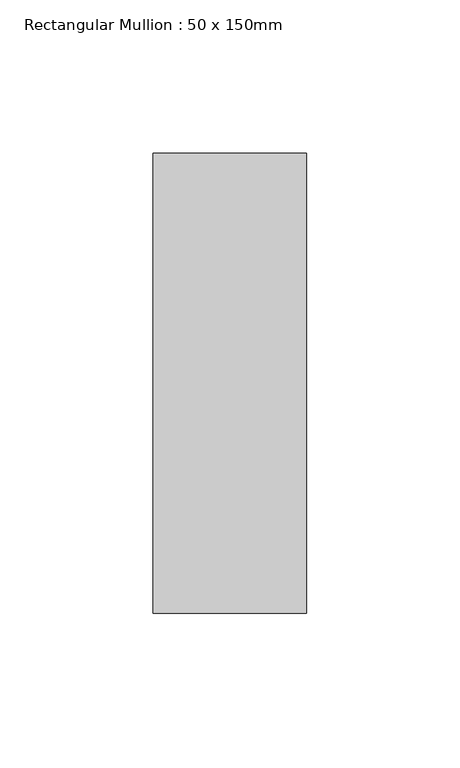
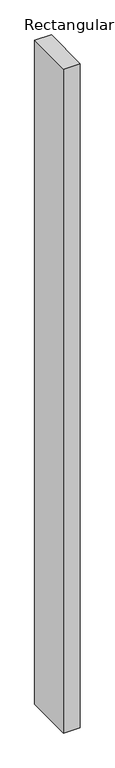
"""IFC4 building model written with IfcOpenShell, lengths in millimetres: member geometry, Rectangular Mullion : 50 x 150mm."""

import ifcopenshell
import ifcopenshell.guid

model = None  # the IFC model being written
_history = None  # IfcOwnerHistory: only IFC2X3 demands one
_inside = {}  # id of a spatial element -> (the spatial element, [elements in it])
_under = {}  # id of a project, library or spatial element -> (it, [spatial elements below it])
_declared = {}  # id of a project -> (the project, [libraries it declares])
_typed = {}  # id of a type object -> (the type object, [elements of that type])
_made_of = {}  # id of a material, layer set ... -> (it, [elements and type objects made of it])


def new_model(schema):
    """Start an empty IFC model of exactly this schema.

    Asked for "IFC4X3", IfcOpenShell would pick the latest addendum, in which some entities
    have other attributes; the version numbers below select the first issue.
    IFC2X3 requires an IfcOwnerHistory on every rooted entity: one is made here for all.
    """
    global model, _history
    if schema == "IFC4X3":
        model = ifcopenshell.file(schema_version=(4, 3, 0, 0))
    else:
        model = ifcopenshell.file(schema=schema)
    _inside.clear()
    _under.clear()
    _declared.clear()
    _typed.clear()
    _made_of.clear()
    _history = None
    if model.schema == "IFC2X3":
        org = make("IfcOrganization", Name="unknown")
        user = make(
            "IfcPersonAndOrganization",
            ThePerson=make("IfcPerson", FamilyName="unknown"),
            TheOrganization=org,
        )
        app = make(
            "IfcApplication",
            ApplicationDeveloper=org,
            Version="unknown",
            ApplicationFullName="unknown",
            ApplicationIdentifier="unknown",
        )
        _history = make(
            "IfcOwnerHistory",
            OwningUser=user,
            OwningApplication=app,
            ChangeAction="ADDED",
            CreationDate=0,
        )
    return model


def make(cls, **values):
    """One entity of the class cls with the attributes given. An attribute that is None is left unset."""
    return model.create_entity(
        cls, **{name: value for name, value in values.items() if value is not None}
    )


def rooted(cls, **values):
    """An entity with a GlobalId (a new one), such as an element, a storey or a relation."""
    return make(cls, GlobalId=ifcopenshell.guid.new(), OwnerHistory=_history, **values)


def si_unit(unit_type, name, prefix=None):
    """IfcSIUnit, for example si_unit("LENGTHUNIT", "METRE", prefix="MILLI")."""
    return make("IfcSIUnit", UnitType=unit_type, Prefix=prefix, Name=name)


def assignment(units):
    """IfcUnitAssignment: the units of a project."""
    return None if units is None else make("IfcUnitAssignment", Units=units)


def point(xyz):
    """IfcCartesianPoint."""
    return None if xyz is None else make("IfcCartesianPoint", Coordinates=xyz)


def direction(xyz):
    """IfcDirection."""
    return None if xyz is None else make("IfcDirection", DirectionRatios=xyz)


def frame(location, z_axis=None, x_axis=None):
    """IfcAxis2Placement3D, a coordinate frame: its origin and axes. An axis left out is left unset."""
    return make(
        "IfcAxis2Placement3D",
        Location=point(location),
        Axis=direction(z_axis),
        RefDirection=direction(x_axis),
    )


def origin():
    """The frame at (0, 0, 0) with its axes left unset."""
    return frame((0.0, 0.0, 0.0))


def place(relative_to, where):
    """IfcLocalPlacement: puts the frame where relative to a parent placement (None: the world)."""
    return make(
        "IfcLocalPlacement", PlacementRelTo=relative_to, RelativePlacement=where
    )


def context(
    kind, dimensions, precision=None, world=None, true_north=None, identifier=None
):
    """IfcGeometricRepresentationContext, for example the 3D "Model" context."""
    return make(
        "IfcGeometricRepresentationContext",
        ContextIdentifier=identifier,
        ContextType=kind,
        CoordinateSpaceDimension=dimensions,
        Precision=precision,
        WorldCoordinateSystem=world,
        TrueNorth=true_north,
    )


def project(units=None, contexts=None):
    """IfcProject with its units and contexts."""
    return rooted(
        "IfcProject",
        Name="project",
        RepresentationContexts=contexts,
        UnitsInContext=assignment(units),
    )


def spatial(cls, under=None, at=None, **own):
    """A site, building, storey or space (cls), placed at a placement, below another one or the project."""
    s = rooted(cls, ObjectPlacement=at, **own)
    if under is not None:
        _under.setdefault(under.id(), (under, []))[1].append(s)
    return s


def polyline(points):
    """IfcPolyline through the points."""
    return make("IfcPolyline", Points=[point(p) for p in points])


def outline(outer, holes=None, kind="AREA"):
    """IfcArbitraryClosedProfileDef: a profile drawn as a closed curve; with holes, ...WithVoids."""
    if holes is None:
        return make("IfcArbitraryClosedProfileDef", ProfileType=kind, OuterCurve=outer)
    return make(
        "IfcArbitraryProfileDefWithVoids",
        ProfileType=kind,
        OuterCurve=outer,
        InnerCurves=holes,
    )


def extrude(swept, where, along, depth):
    """IfcExtrudedAreaSolid: the profile swept, set in the frame where, extruded along a direction by depth."""
    return make(
        "IfcExtrudedAreaSolid",
        SweptArea=swept,
        Position=where,
        ExtrudedDirection=direction(along),
        Depth=depth,
    )


def shape(context_of_items, identifier, shape_type, items):
    """IfcShapeRepresentation: the items that make up one representation, for example the "Body"."""
    return make(
        "IfcShapeRepresentation",
        ContextOfItems=context_of_items,
        RepresentationIdentifier=identifier,
        RepresentationType=shape_type,
        Items=items,
    )


def source(mapping_origin, context_of_items, identifier, shape_type, items):
    """IfcRepresentationMap: a shape defined once, which mapped items show again and again."""
    return make(
        "IfcRepresentationMap",
        MappingOrigin=mapping_origin,
        MappedRepresentation=shape(context_of_items, identifier, shape_type, items),
    )


def transform(
    local_origin,
    x_axis=None,
    y_axis=None,
    z_axis=None,
    scale=None,
    scale2=None,
    scale3=None,
    uniform=True,
):
    """IfcCartesianTransformationOperator3D, or its non-uniform kind. x_axis, y_axis, z_axis: its Axis1, 2, 3."""
    if uniform:
        return make(
            "IfcCartesianTransformationOperator3D",
            Axis1=direction(x_axis),
            Axis2=direction(y_axis),
            LocalOrigin=point(local_origin),
            Scale=scale,
            Axis3=direction(z_axis),
        )
    return make(
        "IfcCartesianTransformationOperator3DnonUniform",
        Axis1=direction(x_axis),
        Axis2=direction(y_axis),
        LocalOrigin=point(local_origin),
        Scale=scale,
        Axis3=direction(z_axis),
        Scale2=scale2,
        Scale3=scale3,
    )


def mapped(mapping_source, mapping_target):
    """IfcMappedItem: shows the shape of a source again, moved by a transform."""
    return make(
        "IfcMappedItem", MappingSource=mapping_source, MappingTarget=mapping_target
    )


def made_of(thing, what):
    """Note that an element or type object is made of a material, layer set ...; save() writes the relation."""
    if what is not None:
        _made_of.setdefault(what.id(), (what, []))[1].append(thing)
    return thing


def element(
    cls,
    number,
    at=None,
    inside=None,
    cuts=None,
    type_object=None,
    material=None,
    context=None,
    identifier="Body",
    shape_type=None,
    held_by="IfcProductDefinitionShape",
    body=None,
    shapes=None,
    **own,
):
    """One element of the class cls, such as IfcWall. Its Tag is "e" and its number.

    at: its placement. inside: the storey or other place that contains it. cuts: it is an
    opening in that element (IfcRelVoidsElement). A single representation is given by context,
    identifier, shape_type and body (its items); several are given by shapes. held_by: the class
    of the entity that holds the representations. save() writes the other relations.
    """
    e = rooted(cls, Tag="e%d" % number, ObjectPlacement=at, **own)
    if body is not None:
        shapes = [shape(context, identifier, shape_type, body)]
    if shapes is not None:
        e.Representation = make(held_by, Representations=shapes)
    if inside is not None:
        _inside.setdefault(inside.id(), (inside, []))[1].append(e)
    if cuts is not None:
        rooted(
            "IfcRelVoidsElement", RelatingBuildingElement=cuts, RelatedOpeningElement=e
        )
    if type_object is not None:
        _typed.setdefault(type_object.id(), (type_object, []))[1].append(e)
    return made_of(e, material)


def aggregate(whole, parts):
    """IfcRelAggregates: a whole, such as a stair, and the parts it consists of."""
    return rooted("IfcRelAggregates", RelatingObject=whole, RelatedObjects=parts)


def save(model, path):
    """Write the relations noted so far, then the file.

    IfcRelAggregates (storeys below a building ...), IfcRelContainedInSpatialStructure (elements
    in a storey), IfcRelDefinesByType, IfcRelAssociatesMaterial and IfcRelDeclares: one each for
    every whole, place, type object, material and project.
    """
    for whole, parts in _under.values():
        aggregate(whole, parts)
    for where, things in _inside.values():
        rooted(
            "IfcRelContainedInSpatialStructure",
            RelatedElements=things,
            RelatingStructure=where,
        )
    for kind, things in _typed.values():
        rooted("IfcRelDefinesByType", RelatedObjects=things, RelatingType=kind)
    for what, things in _made_of.values():
        rooted("IfcRelAssociatesMaterial", RelatedObjects=things, RelatingMaterial=what)
    for by, libraries in _declared.values():
        rooted("IfcRelDeclares", RelatingContext=by, RelatedDefinitions=libraries)
    model.write(path)


def rectangular_mullion_50_x_150mm_2d9f00d1(model_context):
    return source(origin(), model_context, "Body", "SweptSolid", [
        extrude(outline(polyline([(25.0, 75.0), (25.0, -75.0), (-25.0, -75.0), (-25.0, 75.0), (25.0, 75.0)])), frame((0.0, 0.0, -2105.4462072), z_axis=(0.0, 0.0, 1.0), x_axis=(1.0, 0.0, 0.0)), (0.0, 0.0, 1.0), 2105.4462072),
    ])


if __name__ == "__main__":
    model = new_model("IFC4")
    model_context = context("Model", 3, world=origin())
    ifc_project = project(units=[si_unit("LENGTHUNIT", "METRE", prefix="MILLI")], contexts=[model_context])
    site = spatial("IfcSite", under=ifc_project)
    building = spatial("IfcBuilding", under=site)
    placement = place(None, origin())
    rectangular_mullion_50_x_150mm_shape = rectangular_mullion_50_x_150mm_2d9f00d1(model_context)
    element("IfcMember", 1, ObjectType="Rectangular Mullion : 50 x 150mm", at=placement, inside=building, context=model_context, shape_type="MappedRepresentation", body=[
        mapped(rectangular_mullion_50_x_150mm_shape, transform((0.0, 0.0, 0.0), x_axis=(1.0, 0.0, 0.0), y_axis=(0.0, 1.0, 0.0), z_axis=(0.0, 0.0, 1.0))),
    ])
    save(model, "model.ifc")

# Revit data of these elements
# Type "Rectangular Mullion : 50 x 150mm"
#   built-in parameter 1007304 = 0.492126 (stored number, unit not read)
#   built-in parameter 1007301 = 0.082021 (stored number, unit not read)
#   built-in parameter 1007300 = 0.082021 (stored number, unit not read)
# Element 1 (IfcMember, "Rectangular Mullion : 50 x 150mm")
#   Materials on its faces: "Aluminium"
# Materials
#   "Aluminium": class "Metal", colour RGB 247 247 247, transparency 0, Description = "Aluminium 6061", Cost = 0
